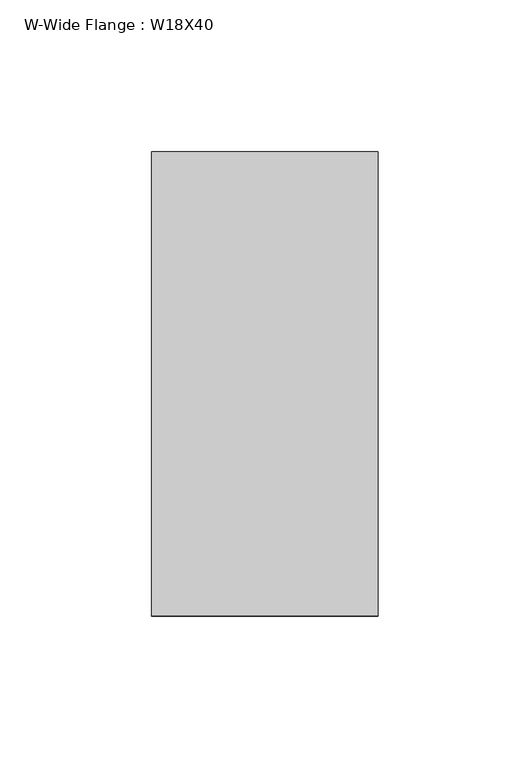
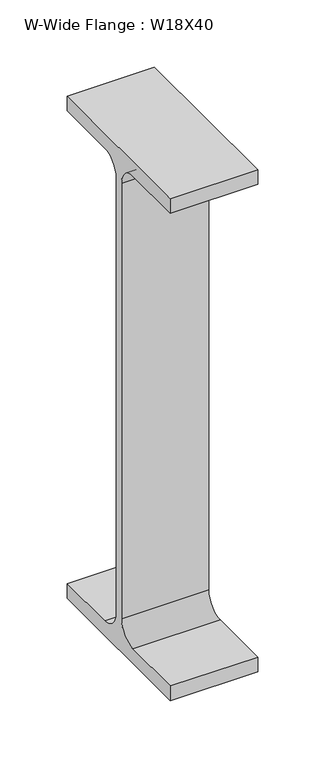
"""IFC4 building model written with IfcOpenShell, lengths in millimetres: beam geometry, W-Wide Flange : W18X40."""

from ifc_helpers import new_model, si_unit, point, frame, frame_2d, origin, place, context, project, spatial, polyline, circle_curve, trimmed, segment, composite_curve, outline, extrude, source, transform, mapped, element, save


def w_wide_flange_w18x40_776be871(model_context):
    return source(origin(), model_context, "Body", "SweptSolid", [
        extrude(outline(composite_curve([segment(polyline([(76.454, -213.995), (76.454, -227.33), (-76.454, -227.33), (-76.454, -213.995), (-20.828, -213.995)]), True, "CONTINUOUS"), segment(trimmed(circle_curve(frame_2d((-20.828, -197.1675)), 16.8275), [point((-20.828, -213.995))], [point((-4.0005, -197.1675))], True, "CARTESIAN"), True, "CONTINUOUS"), segment(polyline([(-4.0005, -197.1675), (-4.0005, 197.1675)]), True, "CONTINUOUS"), segment(trimmed(circle_curve(frame_2d((-20.828, 197.1675)), 16.8275), [point((-4.0005, 197.1675))], [point((-20.828, 213.995))], True, "CARTESIAN"), True, "CONTINUOUS"), segment(polyline([(-20.828, 213.995), (-76.454, 213.995), (-76.454, 227.33), (76.454, 227.33), (76.454, 213.995), (20.828, 213.995)]), True, "CONTINUOUS"), segment(trimmed(circle_curve(frame_2d((20.828, 197.1675)), 16.8275), [point((20.828, 213.995))], [point((4.0005, 197.1675))], True, "CARTESIAN"), True, "CONTINUOUS"), segment(polyline([(4.0005, 197.1675), (4.0005, -197.1675)]), True, "CONTINUOUS"), segment(trimmed(circle_curve(frame_2d((20.828, -197.1675)), 16.8275), [point((4.0005, -197.1675))], [point((20.828, -213.995))], True, "CARTESIAN"), True, "CONTINUOUS"), segment(polyline([(20.828, -213.995), (76.454, -213.995)]), True, "CONTINUOUS")], self_intersect=False)), frame((-68.2625, 0.0, 0.0), z_axis=(1.0, 0.0, 0.0), x_axis=(0.0, 1.0, 0.0)), (0.0, 0.0, 1.0), 74.6125),
    ])


if __name__ == "__main__":
    model = new_model("IFC4")
    model_context = context("Model", 3, world=origin())
    ifc_project = project(units=[si_unit("LENGTHUNIT", "METRE", prefix="MILLI")], contexts=[model_context])
    site = spatial("IfcSite", under=ifc_project)
    building = spatial("IfcBuilding", under=site)
    placement = place(None, origin())
    w_wide_flange_w18x40_shape = w_wide_flange_w18x40_776be871(model_context)
    element("IfcBeam", 1, ObjectType="W-Wide Flange : W18X40", at=placement, inside=building, context=model_context, shape_type="MappedRepresentation", body=[
        mapped(w_wide_flange_w18x40_shape, transform((0.0, 0.0, 0.0), x_axis=(1.0, 0.0, 0.0), y_axis=(0.0, 1.0, 0.0), z_axis=(0.0, 0.0, 1.0))),
    ])
    save(model, "model.ifc")

# Revit data of these elements
# Type "W-Wide Flange : W18X40"
#   Assembly Code = "B10"
#   W = 40
#   Length [instance default] = 5' - 0"
#   bf = 0' - 6.02"
#   d = 1' - 5.9"
#   k = 0' - 1 3/16"
#   k2 = 0' - 0.6625"
#   tf = 0' - 0.525"
#   tw = 0' - 0.315"
#   A = 0.0819444 SF
#   Structural Material [instance default] = Steel ASTM A992
# Element 1 (IfcBeam, "W-Wide Flange : W18X40")
#   Materials on its faces: "Steel ASTM A992"
# Materials
#   "Steel ASTM A992": class "Metal", colour RGB 199 199 199, transparency 0, Description = "Structural steel 50ksi", Cost = 0
